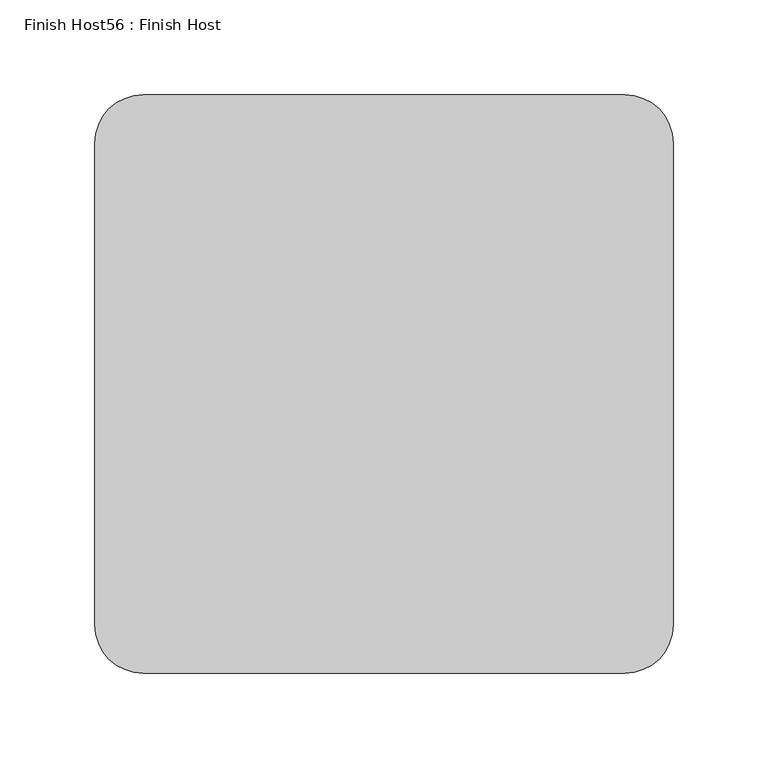
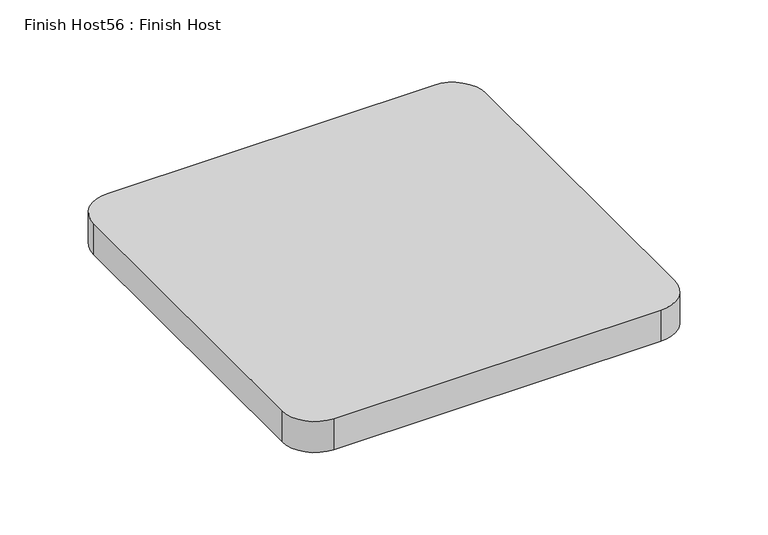
"""IFC4 building model written with IfcOpenShell, lengths in millimetres: proxy geometry, Finish Host56 : Finish Host."""

from ifc_helpers import new_model, si_unit, point, frame_2d, origin, origin_with_axes, place, context, project, spatial, polyline, circle_curve, trimmed, segment, composite_curve, outline, extrude, source, transform, mapped, element, save


def finish_host56_finish_host_0e1f8a48(model_context):
    return source(origin(), model_context, "Body", "SweptSolid", [
        extrude(outline(composite_curve([segment(polyline([(-14217.6939795, 12994.4419385), (-14217.6939795, 13248.4419385)]), True, "CONTINUOUS"), segment(trimmed(circle_curve(frame_2d((-14192.2939795, 13248.4419385)), 25.4), [point((-14217.6939795, 13248.4419385))], [point((-14192.2939795, 13273.8419385))], False, "CARTESIAN"), True, "CONTINUOUS"), segment(polyline([(-14192.2939795, 13273.8419385), (-13938.2939795, 13273.8419385)]), True, "CONTINUOUS"), segment(trimmed(circle_curve(frame_2d((-13938.2939795, 13248.4419385)), 25.4), [point((-13938.2939795, 13273.8419385))], [point((-13912.8939795, 13248.4419385))], False, "CARTESIAN"), True, "CONTINUOUS"), segment(polyline([(-13912.8939795, 13248.4419385), (-13912.8939795, 12994.4419385)]), True, "CONTINUOUS"), segment(trimmed(circle_curve(frame_2d((-13938.2939795, 12994.4419385)), 25.4), [point((-13912.8939795, 12994.4419385))], [point((-13938.2939795, 12969.0419385))], False, "CARTESIAN"), True, "CONTINUOUS"), segment(polyline([(-13938.2939795, 12969.0419385), (-14192.2939795, 12969.0419385)]), True, "CONTINUOUS"), segment(trimmed(circle_curve(frame_2d((-14192.2939795, 12994.4419385)), 25.4), [point((-14192.2939795, 12969.0419385))], [point((-14217.6939795, 12994.4419385))], False, "CARTESIAN"), True, "CONTINUOUS")], self_intersect=False)), origin_with_axes(), (0.0, 0.0, 1.0), 25.4),
    ])


if __name__ == "__main__":
    model = new_model("IFC4")
    model_context = context("Model", 3, world=origin())
    ifc_project = project(units=[si_unit("LENGTHUNIT", "METRE", prefix="MILLI")], contexts=[model_context])
    site = spatial("IfcSite", under=ifc_project)
    building = spatial("IfcBuilding", under=site)
    placement = place(None, origin())
    finish_host56_finish_host_shape = finish_host56_finish_host_0e1f8a48(model_context)
    element("IfcBuildingElementProxy", 1, Name="Finish Host56 : Finish Host", ObjectType="Finish Host56 : Finish Host", at=placement, inside=building, context=model_context, shape_type="MappedRepresentation", body=[
        mapped(finish_host56_finish_host_shape, transform((0.0, 0.0, 0.0), x_axis=(1.0, 0.0, 0.0), y_axis=(0.0, 1.0, 0.0), z_axis=(0.0, 0.0, 1.0))),
    ])
    save(model, "model.ifc")

# Revit data of these elements
# Type "Finish Host56 : Finish Host"
#   Panel Material = none
# Element 1 (IfcBuildingElementProxy, "Finish Host56 : Finish Host")
#   Materials on its faces: "Thread - Teknion - Scarlet"
# Materials
#   "Thread - Teknion - Scarlet": class "Fabric", colour RGB 157 16 25, transparency 0, Model = "F206", Manufacturer = "Teknion Studio", URL = "http://www.teknion.com/", Description = "Fantasme Full Wool", Cost = 0
